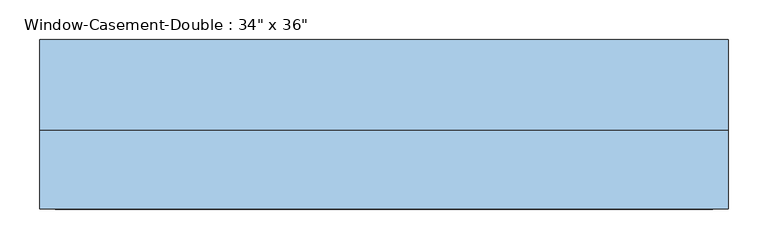
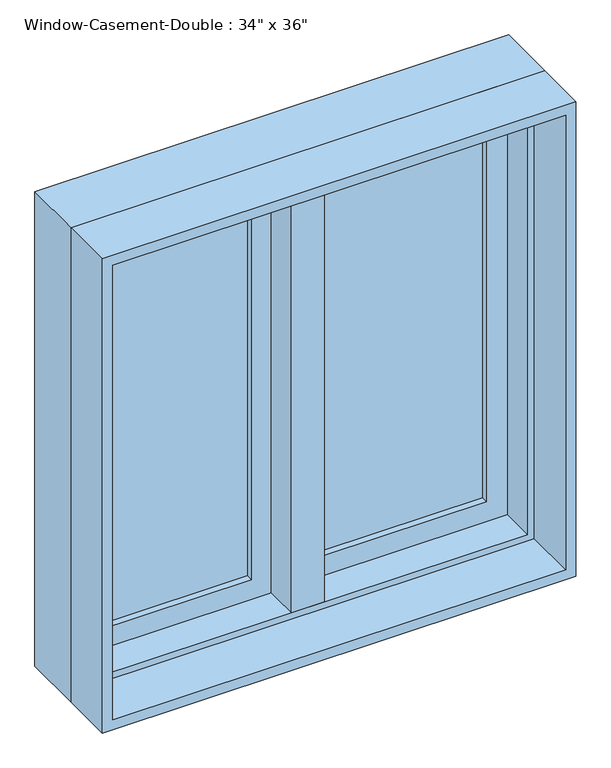
"""IFC4 building model written with IfcOpenShell, lengths in millimetres: window geometry."""

from ifc_helpers import new_model, si_unit, frame, origin, place, context, project, spatial, polyline, outline, extrude, faceted_brep, source, transform, mapped, element, save


def window_4d9d7b27(model_context):
    return source(origin(), model_context, "Body", "SolidModel", [
        faceted_brep([(9.525, 115.8875, 1816.1), (-9.525, 115.8875, 1816.1), (-9.525, 65.0875, 1816.1), (9.525, 65.0875, 1816.1), (9.525, 115.8875, 927.1), (9.525, 65.0875, 927.1), (-9.525, 65.0875, 927.1), (-9.525, 115.8875, 927.1), (-9.525, 65.0875, 946.15), (-9.525, 65.0875, 1797.05), (-30.1625, 65.0875, 946.15), (-30.1625, 65.0875, 1797.05), (-30.1625, 1.5875, 946.15), (-30.1625, 1.5875, 1797.05), (30.1625, 1.5875, 946.15), (30.1625, 1.5875, 1797.05), (30.1625, 65.0875, 946.15), (30.1625, 65.0875, 1797.05), (9.525, 65.0875, 946.15), (9.525, 65.0875, 1797.05)], [[[0, 1, 2, 3]], [[4, 5, 6, 7]], [[1, 0, 4, 7]], [[2, 1, 7, 6, 8, 9]], [[9, 8, 10, 11]], [[11, 10, 12, 13]], [[13, 12, 14, 15]], [[15, 14, 16, 17]], [[17, 16, 18, 19]], [[0, 3, 19, 18, 5, 4]], [[18, 8, 6, 5]], [[9, 19, 3, 2]], [[8, 18, 16, 14, 12, 10]], [[19, 9, 11, 13, 15, 17]]]),
        extrude(outline(polyline([(-66.675, 96.8375), (-66.675, 90.4875), (-361.95, 90.4875), (-361.95, 96.8375), (-66.675, 96.8375)])), frame((0.0, 0.0, 984.25), z_axis=(0.0, 0.0, 1.0), x_axis=(1.0, 0.0, 0.0)), (0.0, 0.0, 1.0), 774.7),
        extrude(outline(polyline([(-361.95, 77.7875), (-361.95, 84.1375), (-66.675, 84.1375), (-66.675, 77.7875), (-361.95, 77.7875)])), frame((0.0, 0.0, 984.25), z_axis=(0.0, 0.0, 1.0), x_axis=(1.0, 0.0, 0.0)), (0.0, 0.0, 1.0), 774.7),
        extrude(outline(polyline([(361.95, 96.8375), (361.95, 90.4875), (66.675, 90.4875), (66.675, 96.8375), (361.95, 96.8375)])), frame((0.0, 0.0, 984.25), z_axis=(0.0, 0.0, 1.0), x_axis=(1.0, 0.0, 0.0)), (0.0, 0.0, 1.0), 774.7),
        extrude(outline(polyline([(66.675, 77.7875), (66.675, 84.1375), (361.95, 84.1375), (361.95, 77.7875), (66.675, 77.7875)])), frame((0.0, 0.0, 984.25), z_axis=(0.0, 0.0, 1.0), x_axis=(1.0, 0.0, 0.0)), (0.0, 0.0, 1.0), 774.7),
        extrude(outline(polyline([(1816.1, -419.1), (927.1, -419.1), (927.1, -9.525), (1816.1, -9.525), (1816.1, -419.1)]), holes=[polyline([(1758.95, -66.675), (984.25, -66.675), (984.25, -361.95), (1758.95, -361.95), (1758.95, -66.675)])]), frame((0.0, 65.0875, 0.0), z_axis=(0.0, 1.0, 0.0), x_axis=(0.0, 0.0, 1.0)), (0.0, 0.0, 1.0), 44.45),
        extrude(outline(polyline([(927.1, 419.1), (1816.1, 419.1), (1816.1, 9.525), (927.1, 9.525), (927.1, 419.1)]), holes=[polyline([(984.25, 66.675), (1758.95, 66.675), (1758.95, 361.95), (984.25, 361.95), (984.25, 66.675)])]), frame((0.0, 65.0875, 0.0), z_axis=(0.0, 1.0, 0.0), x_axis=(0.0, 0.0, 1.0)), (0.0, 0.0, 1.0), 44.45),
        extrude(outline(polyline([(1828.8, -431.8), (914.4, -431.8), (914.4, 431.8), (1828.8, 431.8), (1828.8, -431.8)]), holes=[polyline([(1809.75, 412.75), (933.45, 412.75), (933.45, -412.75), (1809.75, -412.75), (1809.75, 412.75)])]), frame((0.0, -96.8375, 0.0), z_axis=(0.0, 1.0, 0.0), x_axis=(0.0, 0.0, 1.0)), (0.0, 0.0, 1.0), 98.425),
        faceted_brep([(400.05, 65.0875, 1797.05), (400.05, 1.5875, 1797.05), (-400.05, 1.5875, 1797.05), (-400.05, 65.0875, 1797.05), (419.1, 115.8875, 1816.1), (419.1, 65.0875, 1816.1), (-419.1, 65.0875, 1816.1), (-419.1, 115.8875, 1816.1), (431.8, 1.5875, 1828.8), (431.8, 115.8875, 1828.8), (-431.8, 115.8875, 1828.8), (-431.8, 1.5875, 1828.8), (-400.05, 1.5875, 946.15), (-400.05, 65.0875, 946.15), (-419.1, 65.0875, 927.1), (-419.1, 115.8875, 927.1), (-431.8, 115.8875, 914.4), (-431.8, 1.5875, 914.4), (400.05, 1.5875, 946.15), (400.05, 65.0875, 946.15), (419.1, 65.0875, 927.1), (419.1, 115.8875, 927.1), (431.8, 115.8875, 914.4), (431.8, 1.5875, 914.4)], [[[0, 1, 2, 3]], [[4, 5, 6, 7]], [[8, 9, 10, 11]], [[3, 2, 12, 13]], [[7, 6, 14, 15]], [[11, 10, 16, 17]], [[13, 12, 18, 19]], [[15, 14, 20, 21]], [[17, 16, 22, 23]], [[11, 17, 23, 8], [1, 18, 12, 2]], [[19, 18, 1, 0]], [[5, 20, 14, 6], [3, 13, 19, 0]], [[21, 20, 5, 4]], [[23, 22, 9, 8]], [[9, 22, 16, 10], [7, 15, 21, 4]]]),
    ])


if __name__ == "__main__":
    model = new_model("IFC4")
    model_context = context("Model", 3, world=origin())
    ifc_project = project(units=[si_unit("LENGTHUNIT", "METRE", prefix="MILLI")], contexts=[model_context])
    site = spatial("IfcSite", under=ifc_project)
    building = spatial("IfcBuilding", under=site)
    placement = place(None, origin())
    window_shape = window_4d9d7b27(model_context)
    element("IfcWindow", 1, ObjectType="Window-Casement-Double : 34\" x 36\"", at=placement, inside=building, context=model_context, shape_type="MappedRepresentation", body=[
        mapped(window_shape, transform((0.0, 0.0, 0.0), x_axis=(1.0, 0.0, 0.0), y_axis=(0.0, 1.0, 0.0), z_axis=(0.0, 0.0, 1.0))),
    ])
    save(model, "model.ifc")

# Revit data of these elements
# Type "Window-Casement-Double : 34\" x 36\""
#   Type Mark = "59"
#   Fire Rating = "0.5h"
#   Assembly Code = "B2020100"
#   Analytic Construction = "Double glazing - domestic"
#   Frame Extension [instance default] = 0' - 0 1/4"
#   Window Inset [instance default] = 0' - 0"
#   Wall Thickness [instance default] = 0' - 6"
#   Interior Wall Closure [instance default] = 0' - 2 1/4"
#   Half Width = 1' - 5"
#   Visual Light Transmittance = 0.81
#   Thermal Resistance (R) = 1.8146 (h·ft²·°F)/BTU
#   Solar Heat Gain Coefficient = 0.76
#   Rough Width = 2' - 10 1/2"
#   Rough Height = 3' - 0 1/2"
#   Height = 3' - 0"
#   Heat Transfer Coefficient (U) = 0.5511 BTU/(h·ft²·°F)
#   Exterior Wall Closure [instance default] = 0' - 1 1/4"
#   Extension Jamb [instance default] = 0' - 2 1/4"
#   Default Sill Height = 3' - 0"
#   Width = 2' - 10"
#   Define Thermal Properties by = 0
#   Muntin Visibility = yes
#   Interior Trim Visibility [instance default] = yes
#   Exterior Trim Visibility [instance default] = yes
#   Extension Jamb Visibility [instance default] = yes
#   Interior Trim Material = Wood - Stained
#   Muntin Pattern = Muntin Pattern_2x2 : Muntin Pattern_2x2
#   Interior Trim = Trim-Window-Interior-Flat : Picture Frame
#   Interior Frame Material = Wood - Stained
#   Glass Panel Material = Glass
#   Exterior Trim Material = Clad - White
#   Exterior Trim = Trim-Window-Exterior-Flat : with Sill
#   Exterior Frame Material = Clad - White
#   Wall Closure = (empty or 0)
# Element 1 (IfcWindow, "Window-Casement-Double : 34\" x 36\"")
#   Wall Thickness = 0' - 7 5/8"
#   Extension Jamb = 0' - 3 7/8"
#   Materials on its faces: "Wood - Stained", "Glass", "Clad - White"
# Materials
#   "Wood - Stained": class "Wood", colour RGB 224 178 126, transparency 0, Cost = 0
#   "Glass": class "Glass", colour RGB 236 240 239, transparency 0.5, Description = "Soda Lime Glass", Cost = 0
#   "Clad - White": class "Wood", colour RGB 216 216 204, transparency 0, Cost = 0
